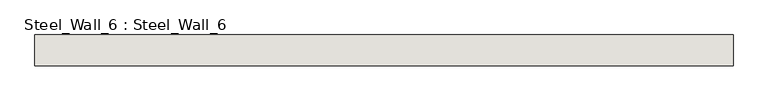
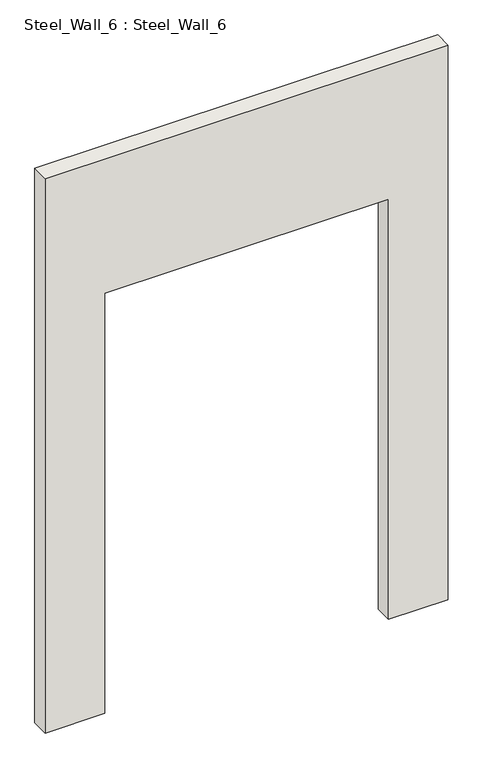
"""IFC4 building model written with IfcOpenShell, lengths in millimetres: wall geometry, Steel_Wall_6 : Steel_Wall_6."""

from ifc_helpers import new_model, si_unit, frame, origin, place, context, project, spatial, polyline, outline, extrude, source, transform, mapped, element, save


def steel_wall_6_steel_wall_6_a34f8d7e(model_context):
    return source(origin(), model_context, "Body", "SweptSolid", [
        extrude(outline(polyline([(3550.0, 2385.0), (3550.0, 115.0), (250.0, 115.0), (250.0, 450.0), (2750.0, 450.0), (2750.0, 2050.0), (250.0, 2050.0), (250.0, 2385.0), (3550.0, 2385.0)])), frame((0.0, 16755.0, 0.0), z_axis=(0.0, 1.0, 0.0), x_axis=(0.0, 0.0, 1.0)), (0.0, 0.0, 1.0), 100.0),
    ])


if __name__ == "__main__":
    model = new_model("IFC4")
    model_context = context("Model", 3, world=origin())
    ifc_project = project(units=[si_unit("LENGTHUNIT", "METRE", prefix="MILLI")], contexts=[model_context])
    site = spatial("IfcSite", under=ifc_project)
    building = spatial("IfcBuilding", under=site)
    placement = place(None, origin())
    steel_wall_6_steel_wall_6_shape = steel_wall_6_steel_wall_6_a34f8d7e(model_context)
    element("IfcWall", 1, ObjectType="Steel_Wall_6 : Steel_Wall_6", at=placement, inside=building, context=model_context, shape_type="MappedRepresentation", body=[
        mapped(steel_wall_6_steel_wall_6_shape, transform((0.0, 0.0, 0.0), x_axis=(1.0, 0.0, 0.0), y_axis=(0.0, 1.0, 0.0), z_axis=(0.0, 0.0, 1.0))),
    ])
    save(model, "model.ifc")

# Revit data of these elements
# Type "Steel_Wall_6 : Steel_Wall_6"
#   NameOverride = "Steel_Wall_6"
# Element 1 (IfcWall, "Steel_Wall_6 : Steel_Wall_6")
#   Materials on its faces: "IfcSurfaceStyle #33"
# Materials
#   "IfcSurfaceStyle #33": class "Unassigned", colour RGB 214 214 214, transparency 0
